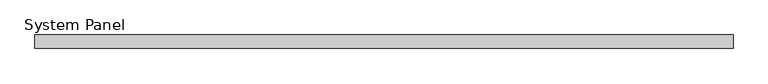
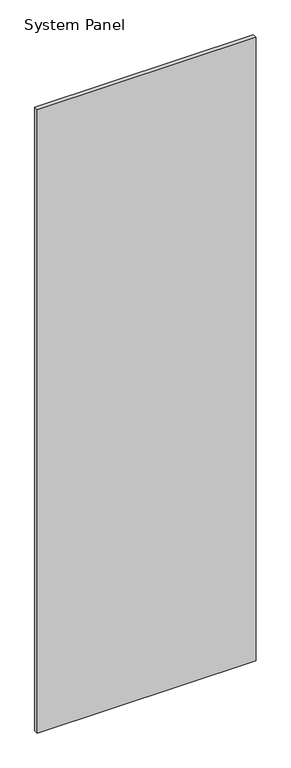
"""IFC4 building model written with IfcOpenShell, lengths in millimetres: plate geometry, System Panel : WWm-Glass-20mm-10mmOffset."""

from ifc_helpers import new_model, si_unit, origin, origin_with_axes, place, context, project, spatial, polyline, outline, extrude, source, transform, mapped, element, save


def system_panel_a5100e41(model_context):
    return source(origin(), model_context, "Body", "SweptSolid", [
        extrude(outline(polyline([(523.4281883, 0.0), (-523.4281883, 0.0), (-523.4281883, 20.0), (523.4281883, 20.0), (523.4281883, 0.0)])), origin_with_axes(), (0.0, 0.0, 1.0), 3150.0),
    ])


if __name__ == "__main__":
    model = new_model("IFC4")
    model_context = context("Model", 3, world=origin())
    ifc_project = project(units=[si_unit("LENGTHUNIT", "METRE", prefix="MILLI")], contexts=[model_context])
    site = spatial("IfcSite", under=ifc_project)
    building = spatial("IfcBuilding", under=site)
    placement = place(None, origin())
    system_panel_shape = system_panel_a5100e41(model_context)
    element("IfcPlate", 1, ObjectType="System Panel : WWm-Glass-20mm-10mmOffset", at=placement, inside=building, context=model_context, shape_type="MappedRepresentation", body=[
        mapped(system_panel_shape, transform((0.0, 0.0, 0.0), x_axis=(1.0, 0.0, 0.0), y_axis=(0.0, 1.0, 0.0), z_axis=(0.0, 0.0, 1.0))),
    ])
    save(model, "model.ifc")

# Revit data of these elements
# Type "System Panel : WWm-Glass-20mm-10mmOffset"
#   Finish = ""
# Element 1 (IfcPlate, "System Panel : WWm-Glass-20mm-10mmOffset")
#   Materials on its faces: "WW-EC-GL-Storefront"
# Materials
#   "WW-EC-GL-Storefront": class "Glass", colour RGB 236 240 239, transparency 0.85, Description = "Storefront Glass", Cost = 0
